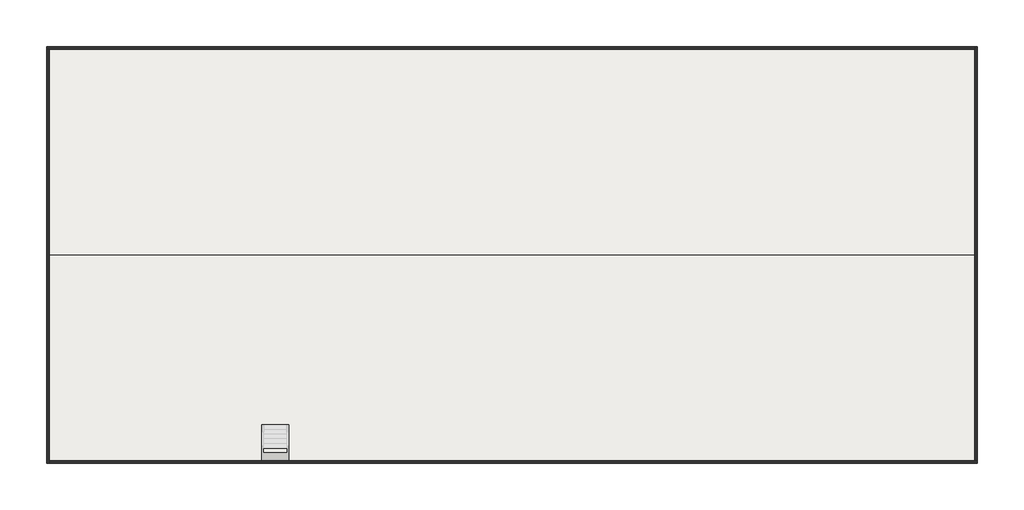
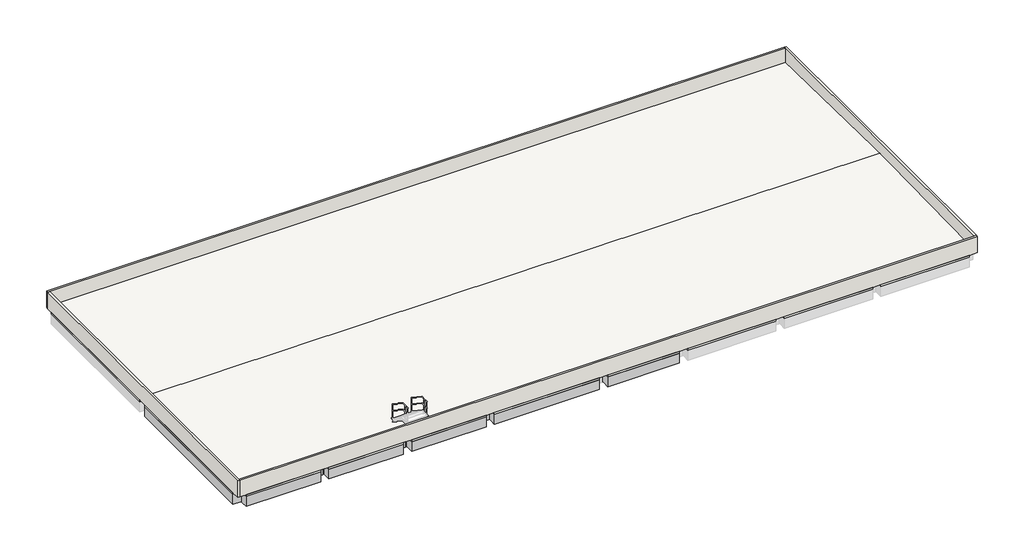
# One storey, part 1 of 3: 16 beams, 4 walls, 1 roof, 1 slab.
"""IFC4 building model written with IfcOpenShell, lengths in millimetres."""

import ifcopenshell
import ifcopenshell.guid

model = None  # the IFC model being written
_history = None  # IfcOwnerHistory: only IFC2X3 demands one
_inside = {}  # id of a spatial element -> (the spatial element, [elements in it])
_under = {}  # id of a project, library or spatial element -> (it, [spatial elements below it])
_declared = {}  # id of a project -> (the project, [libraries it declares])
_typed = {}  # id of a type object -> (the type object, [elements of that type])
_made_of = {}  # id of a material, layer set ... -> (it, [elements and type objects made of it])


def new_model(schema):
    """Start an empty IFC model of exactly this schema.

    Asked for "IFC4X3", IfcOpenShell would pick the latest addendum, in which some entities
    have other attributes; the version numbers below select the first issue.
    IFC2X3 requires an IfcOwnerHistory on every rooted entity: one is made here for all.
    """
    global model, _history
    if schema == "IFC4X3":
        model = ifcopenshell.file(schema_version=(4, 3, 0, 0))
    else:
        model = ifcopenshell.file(schema=schema)
    _inside.clear()
    _under.clear()
    _declared.clear()
    _typed.clear()
    _made_of.clear()
    _history = None
    if model.schema == "IFC2X3":
        org = make("IfcOrganization", Name="unknown")
        user = make(
            "IfcPersonAndOrganization",
            ThePerson=make("IfcPerson", FamilyName="unknown"),
            TheOrganization=org,
        )
        app = make(
            "IfcApplication",
            ApplicationDeveloper=org,
            Version="unknown",
            ApplicationFullName="unknown",
            ApplicationIdentifier="unknown",
        )
        _history = make(
            "IfcOwnerHistory",
            OwningUser=user,
            OwningApplication=app,
            ChangeAction="ADDED",
            CreationDate=0,
        )
    return model


def make(cls, **values):
    """One entity of the class cls with the attributes given. An attribute that is None is left unset."""
    return model.create_entity(
        cls, **{name: value for name, value in values.items() if value is not None}
    )


def rooted(cls, **values):
    """An entity with a GlobalId (a new one), such as an element, a storey or a relation."""
    return make(cls, GlobalId=ifcopenshell.guid.new(), OwnerHistory=_history, **values)


def si_unit(unit_type, name, prefix=None):
    """IfcSIUnit, for example si_unit("LENGTHUNIT", "METRE", prefix="MILLI")."""
    return make("IfcSIUnit", UnitType=unit_type, Prefix=prefix, Name=name)


def assignment(units):
    """IfcUnitAssignment: the units of a project."""
    return None if units is None else make("IfcUnitAssignment", Units=units)


def point(xyz):
    """IfcCartesianPoint."""
    return None if xyz is None else make("IfcCartesianPoint", Coordinates=xyz)


def direction(xyz):
    """IfcDirection."""
    return None if xyz is None else make("IfcDirection", DirectionRatios=xyz)


def frame(location, z_axis=None, x_axis=None):
    """IfcAxis2Placement3D, a coordinate frame: its origin and axes. An axis left out is left unset."""
    return make(
        "IfcAxis2Placement3D",
        Location=point(location),
        Axis=direction(z_axis),
        RefDirection=direction(x_axis),
    )


def origin():
    """The frame at (0, 0, 0) with its axes left unset."""
    return frame((0.0, 0.0, 0.0))


def place(relative_to, where):
    """IfcLocalPlacement: puts the frame where relative to a parent placement (None: the world)."""
    return make(
        "IfcLocalPlacement", PlacementRelTo=relative_to, RelativePlacement=where
    )


def context(
    kind, dimensions, precision=None, world=None, true_north=None, identifier=None
):
    """IfcGeometricRepresentationContext, for example the 3D "Model" context."""
    return make(
        "IfcGeometricRepresentationContext",
        ContextIdentifier=identifier,
        ContextType=kind,
        CoordinateSpaceDimension=dimensions,
        Precision=precision,
        WorldCoordinateSystem=world,
        TrueNorth=true_north,
    )


def project(units=None, contexts=None):
    """IfcProject with its units and contexts."""
    return rooted(
        "IfcProject",
        Name="project",
        RepresentationContexts=contexts,
        UnitsInContext=assignment(units),
    )


def spatial(cls, under=None, at=None, **own):
    """A site, building, storey or space (cls), placed at a placement, below another one or the project."""
    s = rooted(cls, ObjectPlacement=at, **own)
    if under is not None:
        _under.setdefault(under.id(), (under, []))[1].append(s)
    return s


def polyline(points):
    """IfcPolyline through the points."""
    return make("IfcPolyline", Points=[point(p) for p in points])


def outline(outer, holes=None, kind="AREA"):
    """IfcArbitraryClosedProfileDef: a profile drawn as a closed curve; with holes, ...WithVoids."""
    if holes is None:
        return make("IfcArbitraryClosedProfileDef", ProfileType=kind, OuterCurve=outer)
    return make(
        "IfcArbitraryProfileDefWithVoids",
        ProfileType=kind,
        OuterCurve=outer,
        InnerCurves=holes,
    )


def extrude(swept, where, along, depth):
    """IfcExtrudedAreaSolid: the profile swept, set in the frame where, extruded along a direction by depth."""
    return make(
        "IfcExtrudedAreaSolid",
        SweptArea=swept,
        Position=where,
        ExtrudedDirection=direction(along),
        Depth=depth,
    )


def faces_of(points, faces, orient=None, outer=None):
    """IfcFace entities. A face is a list of loops; a loop is a list of indices into points, from 0.

    orient and outer hold one flag for each loop. By default every Orientation is true, the
    first loop of a face is its IfcFaceOuterBound and the others are IfcFaceBound.
    """
    made = []
    for i, loops in enumerate(faces):
        bounds = []
        for j, loop in enumerate(loops):
            is_outer = j == 0 if outer is None else outer[i][j]
            bounds.append(
                make(
                    "IfcFaceOuterBound" if is_outer else "IfcFaceBound",
                    Bound=make("IfcPolyLoop", Polygon=[points[k] for k in loop]),
                    Orientation=True if orient is None else orient[i][j],
                )
            )
        made.append(make("IfcFace", Bounds=bounds))
    return made


def faceted_brep(points, faces, orient=None, outer=None, voids=None):
    """IfcFacetedBrep: a solid bounded by flat faces; with voids (closed shells), ...WithVoids."""
    shared = [point(p) for p in points]
    hull = make("IfcClosedShell", CfsFaces=faces_of(shared, faces, orient, outer))
    if voids is None:
        return make("IfcFacetedBrep", Outer=hull)
    return make(
        "IfcFacetedBrepWithVoids",
        Outer=hull,
        Voids=[
            make(cls, CfsFaces=faces_of(shared, fs, o, b)) for cls, fs, o, b in voids
        ],
    )


def shape(context_of_items, identifier, shape_type, items):
    """IfcShapeRepresentation: the items that make up one representation, for example the "Body"."""
    return make(
        "IfcShapeRepresentation",
        ContextOfItems=context_of_items,
        RepresentationIdentifier=identifier,
        RepresentationType=shape_type,
        Items=items,
    )


def made_of(thing, what):
    """Note that an element or type object is made of a material, layer set ...; save() writes the relation."""
    if what is not None:
        _made_of.setdefault(what.id(), (what, []))[1].append(thing)
    return thing


def element(
    cls,
    number,
    at=None,
    inside=None,
    cuts=None,
    type_object=None,
    material=None,
    context=None,
    identifier="Body",
    shape_type=None,
    held_by="IfcProductDefinitionShape",
    body=None,
    shapes=None,
    **own,
):
    """One element of the class cls, such as IfcWall. Its Tag is "e" and its number.

    at: its placement. inside: the storey or other place that contains it. cuts: it is an
    opening in that element (IfcRelVoidsElement). A single representation is given by context,
    identifier, shape_type and body (its items); several are given by shapes. held_by: the class
    of the entity that holds the representations. save() writes the other relations.
    """
    e = rooted(cls, Tag="e%d" % number, ObjectPlacement=at, **own)
    if body is not None:
        shapes = [shape(context, identifier, shape_type, body)]
    if shapes is not None:
        e.Representation = make(held_by, Representations=shapes)
    if inside is not None:
        _inside.setdefault(inside.id(), (inside, []))[1].append(e)
    if cuts is not None:
        rooted(
            "IfcRelVoidsElement", RelatingBuildingElement=cuts, RelatedOpeningElement=e
        )
    if type_object is not None:
        _typed.setdefault(type_object.id(), (type_object, []))[1].append(e)
    return made_of(e, material)


def aggregate(whole, parts):
    """IfcRelAggregates: a whole, such as a stair, and the parts it consists of."""
    return rooted("IfcRelAggregates", RelatingObject=whole, RelatedObjects=parts)


def save(model, path):
    """Write the relations noted so far, then the file.

    IfcRelAggregates (storeys below a building ...), IfcRelContainedInSpatialStructure (elements
    in a storey), IfcRelDefinesByType, IfcRelAssociatesMaterial and IfcRelDeclares: one each for
    every whole, place, type object, material and project.
    """
    for whole, parts in _under.values():
        aggregate(whole, parts)
    for where, things in _inside.values():
        rooted(
            "IfcRelContainedInSpatialStructure",
            RelatedElements=things,
            RelatingStructure=where,
        )
    for kind, things in _typed.values():
        rooted("IfcRelDefinesByType", RelatedObjects=things, RelatingType=kind)
    for what, things in _made_of.values():
        rooted("IfcRelAssociatesMaterial", RelatedObjects=things, RelatingMaterial=what)
    for by, libraries in _declared.values():
        rooted("IfcRelDeclares", RelatingContext=by, RelatedDefinitions=libraries)
    model.write(path)


model = new_model("IFC4")

# Units and contexts
model_context = context("Model", 3, world=origin())
ifc_project = project(units=[si_unit("LENGTHUNIT", "METRE", prefix="MILLI")], contexts=[model_context])

# Site, building, storey
site = spatial("IfcSite", under=ifc_project)
building = spatial("IfcBuilding", under=site)
storey = spatial("IfcBuildingStorey", under=building, Name="TOC", Elevation=7499.9618634)

# Beams
placement = place(None, origin())
element("IfcBeam", 1, ObjectType="RC Beam_Rectangular : H_SB_AR_S16_B600xH900_RG4", at=placement, inside=storey, context=model_context, shape_type="Brep", body=[
    faceted_brep([(300.0, 12499.5208589, 6599.9618634), (300.0, 12099.5208589, 6599.9618634), (300.0, 11899.5208589, 6599.9618634), (300.0, 11899.5208589, 7349.9618634), (300.0, 12499.5208589, 7349.9618634), (5700.0, 11899.5208589, 6599.9618634), (5700.0, 12099.5208589, 6599.9618634), (5700.0, 12499.5208589, 6599.9618634), (5700.0, 12499.5208589, 7349.9618634), (5700.0, 11899.5208589, 7349.9618634), (426.0, 11899.5208589, 7349.9618634), (2800.0, 11899.5208589, 7349.9618634), (3200.0, 11899.5208589, 7349.9618634), (3200.0, 12499.5208589, 7349.9618634), (2800.0, 12499.5208589, 7349.9618634), (426.0, 12499.5208589, 7349.9618634), (2800.0, 11899.5208589, 6599.9618634), (3200.0, 11899.5208589, 6599.9618634), (426.0, 12499.5208589, 6599.9618634), (2800.0, 12499.5208589, 6599.9618634), (3200.0, 12499.5208589, 6599.9618634)], [[[0, 1, 2, 3, 4]], [[5, 6, 7, 8, 9]], [[4, 3, 10, 11, 12, 9, 8, 13, 14, 15]], [[2, 16, 17, 5, 9, 12, 11, 10, 3]], [[2, 1, 0, 18, 19, 20, 7, 6, 5, 17, 16]], [[7, 20, 19, 18, 0, 4, 15, 14, 13, 8]]]),
])
element("IfcBeam", 2, ObjectType="RC Beam_Rectangular : H_SB_AR_S16_B600xH900_RG4", at=placement, inside=storey, context=model_context, shape_type="Brep", body=[
    faceted_brep([(6300.0, 12499.5208589, 6599.9618634), (6300.0, 12099.5208589, 6599.9618634), (6300.0, 11899.5208589, 6599.9618634), (6300.0, 11899.5208589, 7349.9618634), (6300.0, 12499.5208589, 7349.9618634), (11700.0, 11899.5208589, 6599.9618634), (11700.0, 12099.5208589, 6599.9618634), (11700.0, 12499.5208589, 6599.9618634), (11700.0, 12499.5208589, 7349.9618634), (11700.0, 11899.5208589, 7349.9618634), (8800.0, 11899.5208589, 7349.9618634), (9200.0, 11899.5208589, 7349.9618634), (9200.0, 12499.5208589, 7349.9618634), (8800.0, 12499.5208589, 7349.9618634), (8800.0, 11899.5208589, 6599.9618634), (9200.0, 11899.5208589, 6599.9618634), (8800.0, 12499.5208589, 6599.9618634), (9200.0, 12499.5208589, 6599.9618634)], [[[0, 1, 2, 3, 4]], [[5, 6, 7, 8, 9]], [[4, 3, 10, 11, 9, 8, 12, 13]], [[2, 14, 15, 5, 9, 11, 10, 3]], [[2, 1, 0, 16, 17, 7, 6, 5, 15, 14]], [[7, 17, 16, 0, 4, 13, 12, 8]]]),
])
element("IfcBeam", 3, ObjectType="RC Beam_Rectangular : H_SB_AR_S16_B600xH900_RG4", at=placement, inside=storey, context=model_context, shape_type="Brep", body=[
    faceted_brep([(12300.0, 12499.5208589, 6599.9618634), (12300.0, 12099.5208589, 6599.9618634), (12300.0, 11899.5208589, 6599.9618634), (12300.0, 11899.5208589, 7349.9618634), (12300.0, 12499.5208589, 7349.9618634), (17700.0, 11899.5208589, 6599.9618634), (17700.0, 12099.5208589, 6599.9618634), (17700.0, 12499.5208589, 6599.9618634), (17700.0, 12499.5208589, 7349.9618634), (17700.0, 11899.5208589, 7349.9618634), (14800.0, 11899.5208589, 7349.9618634), (15200.0, 11899.5208589, 7349.9618634), (15200.0, 12499.5208589, 7349.9618634), (14800.0, 12499.5208589, 7349.9618634), (14800.0, 11899.5208589, 6599.9618634), (15200.0, 11899.5208589, 6599.9618634), (14800.0, 12499.5208589, 6599.9618634), (15200.0, 12499.5208589, 6599.9618634)], [[[0, 1, 2, 3, 4]], [[5, 6, 7, 8, 9]], [[4, 3, 10, 11, 9, 8, 12, 13]], [[2, 14, 15, 5, 9, 11, 10, 3]], [[2, 1, 0, 16, 17, 7, 6, 5, 15, 14]], [[7, 17, 16, 0, 4, 13, 12, 8]]]),
])
element("IfcBeam", 4, ObjectType="RC Beam_Rectangular : H_SB_AR_S16_B600xH900_RG9", at=placement, inside=storey, context=model_context, shape_type="Brep", body=[
    faceted_brep([(300.0, 799.5208589, 6599.9618634), (300.0, 649.5208589, 6599.9618634), (300.0, 199.5208589, 6599.9618634), (300.0, 199.5208589, 7349.9618634), (300.0, 799.5208589, 7349.9618634), (5700.0, 199.5208589, 6599.9618634), (5700.0, 649.5208589, 6599.9618634), (5700.0, 799.5208589, 6599.9618634), (5700.0, 799.5208589, 7349.9618634), (5700.0, 199.5208589, 7349.9618634), (3200.0, 799.5208589, 7349.9618634), (2800.0, 799.5208589, 7349.9618634), (426.0, 799.5208589, 7349.9618634), (2800.0, 799.5208589, 6599.9618634), (3200.0, 799.5208589, 6599.9618634)], [[[0, 1, 2, 3, 4]], [[5, 6, 7, 8, 9]], [[4, 3, 9, 8, 10, 11, 12]], [[2, 5, 9, 3]], [[2, 1, 0, 13, 14, 7, 6, 5]], [[7, 14, 13, 0, 4, 12, 11, 10, 8]]]),
])
element("IfcBeam", 5, ObjectType="RC Beam_Rectangular : H_SB_AR_S16_B600xH900_RG9", at=placement, inside=storey, context=model_context, shape_type="Brep", body=[
    faceted_brep([(6300.0, 799.5208589, 6599.9618634), (6300.0, 649.5208589, 6599.9618634), (6300.0, 199.5208589, 6599.9618634), (6300.0, 199.5208589, 7349.9618634), (6300.0, 799.5208589, 7349.9618634), (11700.0, 199.5208589, 6599.9618634), (11700.0, 649.5208589, 6599.9618634), (11700.0, 799.5208589, 6599.9618634), (11700.0, 799.5208589, 7349.9618634), (11700.0, 199.5208589, 7349.9618634), (9200.0, 799.5208589, 7349.9618634), (8800.0, 799.5208589, 7349.9618634), (8800.0, 799.5208589, 6599.9618634), (9200.0, 799.5208589, 6599.9618634)], [[[0, 1, 2, 3, 4]], [[5, 6, 7, 8, 9]], [[4, 3, 9, 8, 10, 11]], [[2, 5, 9, 3]], [[2, 1, 0, 12, 13, 7, 6, 5]], [[7, 13, 12, 0, 4, 11, 10, 8]]]),
])
element("IfcBeam", 6, ObjectType="RC Beam_Rectangular : H_SB_AR_S16_B600xH900_RG9", at=placement, inside=storey, context=model_context, shape_type="Brep", body=[
    faceted_brep([(12300.0, 799.5208589, 6599.9618634), (12300.0, 649.5208589, 6599.9618634), (12300.0, 199.5208589, 6599.9618634), (12300.0, 199.5208589, 7349.9618634), (12300.0, 799.5208589, 7349.9618634), (17700.0, 199.5208589, 6599.9618634), (17700.0, 649.5208589, 6599.9618634), (17700.0, 799.5208589, 6599.9618634), (17700.0, 799.5208589, 7349.9618634), (17700.0, 199.5208589, 7349.9618634), (15200.0, 799.5208589, 7349.9618634), (14800.0, 799.5208589, 7349.9618634), (14800.0, 799.5208589, 6599.9618634), (15200.0, 799.5208589, 6599.9618634)], [[[0, 1, 2, 3, 4]], [[5, 6, 7, 8, 9]], [[4, 3, 9, 8, 10, 11]], [[2, 5, 9, 3]], [[2, 1, 0, 12, 13, 7, 6, 5]], [[7, 13, 12, 0, 4, 11, 10, 8]]]),
])
element("IfcBeam", 7, ObjectType="RC Beam_Rectangular : H_SB_AR_S16_B600xH900_RG9", at=placement, inside=storey, context=model_context, shape_type="Brep", body=[
    faceted_brep([(18300.0, 799.5208589, 6599.9618634), (18300.0, 649.5208589, 6599.9618634), (18300.0, 199.5208589, 6599.9618634), (18300.0, 199.5208589, 7349.9618634), (18300.0, 799.5208589, 7349.9618634), (25900.0, 199.5208589, 6599.9618634), (25900.0, 649.5208589, 6599.9618634), (25900.0, 799.5208589, 6599.9618634), (25900.0, 799.5208589, 7349.9618634), (25900.0, 199.5208589, 7349.9618634), (22400.0, 799.5208589, 7349.9618634), (21800.0, 799.5208589, 7349.9618634), (21800.0, 799.5208589, 6599.9618634), (22400.0, 799.5208589, 6599.9618634)], [[[0, 1, 2, 3, 4]], [[5, 6, 7, 8, 9]], [[4, 3, 9, 8, 10, 11]], [[2, 5, 9, 3]], [[2, 1, 0, 12, 13, 7, 6, 5]], [[7, 13, 12, 0, 4, 11, 10, 8]]]),
])
element("IfcBeam", 8, ObjectType="RC Beam_Rectangular : H_SB_AR_S16_B600xH900_RG9", at=placement, inside=storey, context=model_context, shape_type="Brep", body=[
    faceted_brep([(26500.0, 799.5208589, 6599.9618634), (26500.0, 649.5208589, 6599.9618634), (26500.0, 199.5208589, 6599.9618634), (26500.0, 199.5208589, 7349.9618634), (26500.0, 799.5208589, 7349.9618634), (31700.0, 199.5208589, 6599.9618634), (31700.0, 649.5208589, 6599.9618634), (31700.0, 799.5208589, 6599.9618634), (31700.0, 799.5208589, 7349.9618634), (31700.0, 199.5208589, 7349.9618634), (29400.0, 799.5208589, 7349.9618634), (28800.0, 799.5208589, 7349.9618634), (28700.0, 799.5208589, 7349.9618634), (28500.0, 799.5208589, 7349.9618634), (27855.0, 799.5208589, 7349.9618634), (26724.0, 799.5208589, 7349.9618634), (28800.0, 799.5208589, 6599.9618634), (29400.0, 799.5208589, 6599.9618634)], [[[0, 1, 2, 3, 4]], [[5, 6, 7, 8, 9]], [[4, 3, 9, 8, 10, 11, 12, 13, 14, 15]], [[2, 5, 9, 3]], [[2, 1, 0, 16, 17, 7, 6, 5]], [[7, 17, 16, 0, 4, 15, 14, 13, 12, 11, 10, 8]]]),
])
element("IfcBeam", 9, ObjectType="RC Beam_Rectangular : H_SB_AR_S16_B600xH900_RG6", at=placement, inside=storey, context=model_context, shape_type="Brep", body=[
    faceted_brep([(300.0, 11899.5208589, 6599.9618634), (150.0, 11899.5208589, 6599.9618634), (-300.0, 11899.5208589, 6599.9618634), (-300.0, 11899.5208589, 7349.9618634), (300.0, 11899.5208589, 7349.9618634), (-300.0, 799.5208589, 6599.9618634), (150.0, 799.5208589, 6599.9618634), (300.0, 799.5208589, 6599.9618634), (300.0, 799.5208589, 7349.9618634), (-300.0, 799.5208589, 7349.9618634)], [[[0, 1, 2, 3, 4]], [[5, 6, 7, 8, 9]], [[4, 3, 9, 8]], [[7, 0, 4, 8]], [[2, 1, 0, 7, 6, 5]], [[2, 5, 9, 3]]]),
])
element("IfcBeam", 10, ObjectType="RC Beam_Rectangular : H_SB_AR_S16_B400xH900_RG1", at=placement, inside=storey, context=model_context, shape_type="Brep", body=[
    faceted_brep([(5800.0, 799.5208589, 7349.9618634), (6200.0, 799.5208589, 7349.9618634), (6200.0, 925.5208589, 7349.9618634), (6200.0, 11899.5208589, 7349.9618634), (5800.0, 11899.5208589, 7349.9618634), (5800.0, 925.5208589, 7349.9618634), (5800.0, 799.5208589, 6599.9618634), (6200.0, 799.5208589, 6599.9618634), (6200.0, 11899.5208589, 6599.9618634), (5800.0, 11899.5208589, 6599.9618634), (6200.0, 925.5208589, 6599.9618634), (5800.0, 925.5208589, 6599.9618634)], [[[0, 1, 2, 3, 4, 5]], [[6, 7, 1, 0]], [[8, 9, 4, 3]], [[7, 10, 8, 3, 2, 1]], [[6, 11, 9, 8, 10, 7]], [[9, 11, 6, 0, 5, 4]]]),
])
element("IfcBeam", 11, ObjectType="RC Beam_Rectangular : H_SB_AR_S16_B400xH900_RG1", at=placement, inside=storey, context=model_context, shape_type="Brep", body=[
    faceted_brep([(11800.0, 799.5208589, 7349.9618634), (12200.0, 799.5208589, 7349.9618634), (12200.0, 925.5208589, 7349.9618634), (12200.0, 11899.5208589, 7349.9618634), (11800.0, 11899.5208589, 7349.9618634), (11800.0, 925.5208589, 7349.9618634), (11800.0, 799.5208589, 6599.9618634), (12200.0, 799.5208589, 6599.9618634), (12200.0, 11899.5208589, 6599.9618634), (11800.0, 11899.5208589, 6599.9618634), (12200.0, 925.5208589, 6599.9618634), (11800.0, 925.5208589, 6599.9618634)], [[[0, 1, 2, 3, 4, 5]], [[6, 7, 1, 0]], [[8, 9, 4, 3]], [[7, 10, 8, 3, 2, 1]], [[6, 11, 9, 8, 10, 7]], [[9, 11, 6, 0, 5, 4]]]),
])
element("IfcBeam", 12, ObjectType="RC Beam_Rectangular : H_SB_AR_S16_B600xH900_RG1A", at=placement, inside=storey, context=model_context, shape_type="Brep", body=[
    faceted_brep([(17700.0, 799.5208589, 7349.9618634), (18300.0, 799.5208589, 7349.9618634), (18300.0, 925.5208589, 7349.9618634), (18300.0, 7999.5208589, 7349.9618634), (18300.0, 8599.5208589, 7349.9618634), (18300.0, 11899.5208589, 7349.9618634), (17700.0, 11899.5208589, 7349.9618634), (17700.0, 925.5208589, 7349.9618634), (17700.0, 799.5208589, 6599.9618634), (18100.0, 799.5208589, 6599.9618634), (18300.0, 799.5208589, 6599.9618634), (18300.0, 11899.5208589, 6599.9618634), (18100.0, 11899.5208589, 6599.9618634), (17700.0, 11899.5208589, 6599.9618634), (18300.0, 7999.5208589, 6599.9618634), (18300.0, 8599.5208589, 6599.9618634), (17700.0, 925.5208589, 6599.9618634)], [[[0, 1, 2, 3, 4, 5, 6, 7]], [[8, 9, 10, 1, 0]], [[11, 12, 13, 6, 5]], [[10, 14, 15, 11, 5, 4, 3, 2, 1]], [[8, 16, 13, 12, 11, 15, 14, 10, 9]], [[13, 16, 8, 0, 7, 6]]]),
])
element("IfcBeam", 13, ObjectType="RC Beam_Rectangular : H_SB_AR_S16_B400xH900_RB1", at=placement, inside=storey, context=model_context, shape_type="Brep", body=[
    faceted_brep([(2800.0, 11899.5208589, 6599.9618634), (2800.0, 925.5208589, 6599.9618634), (2800.0, 799.5208589, 6599.9618634), (2800.0, 799.5208589, 7349.9618634), (2800.0, 925.5208589, 7349.9618634), (2800.0, 11899.5208589, 7349.9618634), (3200.0, 11899.5208589, 6599.9618634), (3200.0, 925.5208589, 6599.9618634), (3200.0, 799.5208589, 6599.9618634), (3200.0, 11899.5208589, 7349.9618634), (3200.0, 925.5208589, 7349.9618634), (3200.0, 799.5208589, 7349.9618634)], [[[0, 1, 2, 3, 4, 5]], [[0, 6, 7, 8, 2, 1]], [[8, 7, 6, 9, 10, 11]], [[6, 0, 5, 9]], [[2, 8, 11, 3]], [[5, 4, 3, 11, 10, 9]]]),
])
element("IfcBeam", 14, ObjectType="RC Beam_Rectangular : H_SB_AR_S16_B400xH900_RB1", at=placement, inside=storey, context=model_context, shape_type="Brep", body=[
    faceted_brep([(8800.0, 11899.5208589, 6599.9618634), (8800.0, 925.5208589, 6599.9618634), (8800.0, 799.5208589, 6599.9618634), (8800.0, 799.5208589, 7349.9618634), (8800.0, 925.5208589, 7349.9618634), (8800.0, 11899.5208589, 7349.9618634), (9200.0, 11899.5208589, 6599.9618634), (9200.0, 925.5208589, 6599.9618634), (9200.0, 799.5208589, 6599.9618634), (9200.0, 11899.5208589, 7349.9618634), (9200.0, 925.5208589, 7349.9618634), (9200.0, 799.5208589, 7349.9618634)], [[[0, 1, 2, 3, 4, 5]], [[0, 6, 7, 8, 2, 1]], [[8, 7, 6, 9, 10, 11]], [[6, 0, 5, 9]], [[2, 8, 11, 3]], [[5, 4, 3, 11, 10, 9]]]),
])
element("IfcBeam", 15, ObjectType="RC Beam_Rectangular : H_SB_AR_S16_B400xH900_RB1", at=placement, inside=storey, context=model_context, shape_type="Brep", body=[
    faceted_brep([(14800.0, 11899.5208589, 6599.9618634), (14800.0, 925.5208589, 6599.9618634), (14800.0, 799.5208589, 6599.9618634), (14800.0, 799.5208589, 7349.9618634), (14800.0, 925.5208589, 7349.9618634), (14800.0, 11899.5208589, 7349.9618634), (15200.0, 11899.5208589, 6599.9618634), (15200.0, 925.5208589, 6599.9618634), (15200.0, 799.5208589, 6599.9618634), (15200.0, 11899.5208589, 7349.9618634), (15200.0, 925.5208589, 7349.9618634), (15200.0, 799.5208589, 7349.9618634)], [[[0, 1, 2, 3, 4, 5]], [[0, 6, 7, 8, 2, 1]], [[8, 7, 6, 9, 10, 11]], [[6, 0, 5, 9]], [[2, 8, 11, 3]], [[5, 4, 3, 11, 10, 9]]]),
])
element("IfcBeam", 16, ObjectType="RC Beam_Rectangular : H_SB_AR_S16_B600xH900_RB3", at=placement, inside=storey, context=model_context, shape_type="Brep", body=[
    faceted_brep([(21800.0, 7999.5208589, 6599.9618634), (21800.0, 925.5208589, 6599.9618634), (21800.0, 799.5208589, 6599.9618634), (21800.0, 799.5208589, 7349.9618634), (21800.0, 925.5208589, 7349.9618634), (21800.0, 7999.5208589, 7349.9618634), (22400.0, 7999.5208589, 6599.9618634), (22400.0, 925.5208589, 6599.9618634), (22400.0, 799.5208589, 6599.9618634), (22400.0, 7999.5208589, 7349.9618634), (22400.0, 925.5208589, 7349.9618634), (22400.0, 799.5208589, 7349.9618634)], [[[0, 1, 2, 3, 4, 5]], [[0, 6, 7, 8, 2, 1]], [[8, 7, 6, 9, 10, 11]], [[6, 0, 5, 9]], [[2, 8, 11, 3]], [[5, 4, 3, 11, 10, 9]]]),
])

# Roof
element("IfcRoof", 17, ObjectType="H_RF_AR_B06_Mortar(Slope)_XPS_Memb_T50+120", at=placement, inside=storey, context=model_context, shape_type="SweptSolid", body=[
    extrude(outline(polyline([(24049.5208589, 7671.4618634), (24049.5208589, 7499.9618634), (349.5208589, 7499.9618634), (349.5208589, 7671.4618634), (12199.5208589, 7904.4618634), (24049.5208589, 7671.4618634)])), frame((-150.0, 0.0, 0.0), z_axis=(1.0, 0.0, 0.0), x_axis=(0.0, 1.0, 0.0)), (0.0, 0.0, 1.0), 53300.0),
])

# Slab
element("IfcSlab", 18, ObjectType="H_FL_AR_S17_Roof RC Slab_T150", at=placement, inside=storey, context=model_context, shape_type="Brep", body=[
    faceted_brep([(300.0, 11899.5208589, 7349.9618634), (300.0, 12499.5208589, 7349.9618634), (-300.0, 12499.5208589, 7349.9618634), (-300.0, 23599.5208589, 7349.9618634), (300.0, 23599.5208589, 7349.9618634), (300.0, 24199.5208589, 7349.9618634), (5700.0, 24199.5208589, 7349.9618634), (5700.0, 23599.5208589, 7349.9618634), (5800.0, 23599.5208589, 7349.9618634), (6200.0, 23599.5208589, 7349.9618634), (6300.0, 23599.5208589, 7349.9618634), (6300.0, 24199.5208589, 7349.9618634), (11700.0, 24199.5208589, 7349.9618634), (11700.0, 23599.5208589, 7349.9618634), (11800.0, 23599.5208589, 7349.9618634), (12200.0, 23599.5208589, 7349.9618634), (12300.0, 23599.5208589, 7349.9618634), (12300.0, 24199.5208589, 7349.9618634), (17700.0, 24199.5208589, 7349.9618634), (17700.0, 23599.5208589, 7349.9618634), (18300.0, 23599.5208589, 7349.9618634), (18300.0, 24199.5208589, 7349.9618634), (25900.0, 24199.5208589, 7349.9618634), (25900.0, 23599.5208589, 7349.9618634), (25950.0, 23599.5208589, 7349.9618634), (26450.0, 23599.5208589, 7349.9618634), (26500.0, 23599.5208589, 7349.9618634), (26500.0, 24199.5208589, 7349.9618634), (31700.0, 24199.5208589, 7349.9618634), (31700.0, 23599.5208589, 7349.9618634), (31750.0, 23599.5208589, 7349.9618634), (32250.0, 23599.5208589, 7349.9618634), (32300.0, 23599.5208589, 7349.9618634), (32300.0, 24199.5208589, 7349.9618634), (38700.0, 24199.5208589, 7349.9618634), (38700.0, 23599.5208589, 7349.9618634), (38750.0, 23599.5208589, 7349.9618634), (39250.0, 23599.5208589, 7349.9618634), (39300.0, 23599.5208589, 7349.9618634), (39300.0, 24199.5208589, 7349.9618634), (45700.0, 24199.5208589, 7349.9618634), (45700.0, 23599.5208589, 7349.9618634), (45750.0, 23599.5208589, 7349.9618634), (46250.0, 23599.5208589, 7349.9618634), (46300.0, 23599.5208589, 7349.9618634), (46300.0, 24199.5208589, 7349.9618634), (52700.0, 24199.5208589, 7349.9618634), (52700.0, 23599.5208589, 7349.9618634), (53300.0, 23599.5208589, 7349.9618634), (53300.0, 8599.5208589, 7349.9618634), (52700.0, 8599.5208589, 7349.9618634), (52700.0, 7999.5208589, 7349.9618634), (53300.0, 7999.5208589, 7349.9618634), (53300.0, 799.5208589, 7349.9618634), (52700.0, 799.5208589, 7349.9618634), (52700.0, 199.5208589, 7349.9618634), (46300.0, 199.5208589, 7349.9618634), (46300.0, 799.5208589, 7349.9618634), (46250.0, 799.5208589, 7349.9618634), (45750.0, 799.5208589, 7349.9618634), (45700.0, 799.5208589, 7349.9618634), (45700.0, 199.5208589, 7349.9618634), (39300.0, 199.5208589, 7349.9618634), (39300.0, 799.5208589, 7349.9618634), (39250.0, 799.5208589, 7349.9618634), (38750.0, 799.5208589, 7349.9618634), (38700.0, 799.5208589, 7349.9618634), (38700.0, 199.5208589, 7349.9618634), (32300.0, 199.5208589, 7349.9618634), (32300.0, 799.5208589, 7349.9618634), (32250.0, 799.5208589, 7349.9618634), (31750.0, 799.5208589, 7349.9618634), (31700.0, 799.5208589, 7349.9618634), (31700.0, 199.5208589, 7349.9618634), (26500.0, 199.5208589, 7349.9618634), (26500.0, 799.5208589, 7349.9618634), (26450.0, 799.5208589, 7349.9618634), (25950.0, 799.5208589, 7349.9618634), (25900.0, 799.5208589, 7349.9618634), (25900.0, 199.5208589, 7349.9618634), (18300.0, 199.5208589, 7349.9618634), (18300.0, 799.5208589, 7349.9618634), (17700.0, 799.5208589, 7349.9618634), (17700.0, 199.5208589, 7349.9618634), (12300.0, 199.5208589, 7349.9618634), (12300.0, 799.5208589, 7349.9618634), (12200.0, 799.5208589, 7349.9618634), (11800.0, 799.5208589, 7349.9618634), (11700.0, 799.5208589, 7349.9618634), (11700.0, 199.5208589, 7349.9618634), (6300.0, 199.5208589, 7349.9618634), (6300.0, 799.5208589, 7349.9618634), (6200.0, 799.5208589, 7349.9618634), (5800.0, 799.5208589, 7349.9618634), (5700.0, 799.5208589, 7349.9618634), (5700.0, 199.5208589, 7349.9618634), (300.0, 199.5208589, 7349.9618634), (300.0, 799.5208589, 7349.9618634), (-300.0, 799.5208589, 7349.9618634), (-300.0, 11899.5208589, 7349.9618634), (18300.0, 11899.5208589, 7349.9618634), (18300.0, 12499.5208589, 7349.9618634), (17700.0, 12499.5208589, 7349.9618634), (17700.0, 11899.5208589, 7349.9618634), (6300.0, 11899.5208589, 7349.9618634), (6300.0, 12499.5208589, 7349.9618634), (6200.0, 12499.5208589, 7349.9618634), (5800.0, 12499.5208589, 7349.9618634), (5700.0, 12499.5208589, 7349.9618634), (5700.0, 11899.5208589, 7349.9618634), (5800.0, 11899.5208589, 7349.9618634), (6200.0, 11899.5208589, 7349.9618634), (12300.0, 11899.5208589, 7349.9618634), (12300.0, 12499.5208589, 7349.9618634), (12200.0, 12499.5208589, 7349.9618634), (11800.0, 12499.5208589, 7349.9618634), (11700.0, 12499.5208589, 7349.9618634), (11700.0, 11899.5208589, 7349.9618634), (11800.0, 11899.5208589, 7349.9618634), (12200.0, 11899.5208589, 7349.9618634), (26500.0, 7999.5208589, 7349.9618634), (26500.0, 8599.5208589, 7349.9618634), (26450.0, 8599.5208589, 7349.9618634), (25950.0, 8599.5208589, 7349.9618634), (25900.0, 8599.5208589, 7349.9618634), (25900.0, 7999.5208589, 7349.9618634), (25950.0, 7999.5208589, 7349.9618634), (26450.0, 7999.5208589, 7349.9618634), (32300.0, 7999.5208589, 7349.9618634), (32300.0, 8599.5208589, 7349.9618634), (32250.0, 8599.5208589, 7349.9618634), (31750.0, 8599.5208589, 7349.9618634), (31700.0, 8599.5208589, 7349.9618634), (31700.0, 7999.5208589, 7349.9618634), (31750.0, 7999.5208589, 7349.9618634), (32250.0, 7999.5208589, 7349.9618634), (39300.0, 7999.5208589, 7349.9618634), (39300.0, 8599.5208589, 7349.9618634), (39250.0, 8599.5208589, 7349.9618634), (38750.0, 8599.5208589, 7349.9618634), (38700.0, 8599.5208589, 7349.9618634), (38700.0, 7999.5208589, 7349.9618634), (38750.0, 7999.5208589, 7349.9618634), (39250.0, 7999.5208589, 7349.9618634), (46300.0, 7999.5208589, 7349.9618634), (46300.0, 8599.5208589, 7349.9618634), (46250.0, 8599.5208589, 7349.9618634), (45750.0, 8599.5208589, 7349.9618634), (45700.0, 8599.5208589, 7349.9618634), (45700.0, 7999.5208589, 7349.9618634), (45750.0, 7999.5208589, 7349.9618634), (46250.0, 7999.5208589, 7349.9618634), (300.0, 12499.5208589, 7499.9618634), (300.0, 11899.5208589, 7499.9618634), (-300.0, 11899.5208589, 7499.9618634), (-300.0, 799.5208589, 7499.9618634), (300.0, 799.5208589, 7499.9618634), (300.0, 199.5208589, 7499.9618634), (5700.0, 199.5208589, 7499.9618634), (5700.0, 799.5208589, 7499.9618634), (6300.0, 799.5208589, 7499.9618634), (6300.0, 199.5208589, 7499.9618634), (11700.0, 199.5208589, 7499.9618634), (11700.0, 799.5208589, 7499.9618634), (12300.0, 799.5208589, 7499.9618634), (12300.0, 199.5208589, 7499.9618634), (17700.0, 199.5208589, 7499.9618634), (17700.0, 799.5208589, 7499.9618634), (18300.0, 799.5208589, 7499.9618634), (18300.0, 199.5208589, 7499.9618634), (25900.0, 199.5208589, 7499.9618634), (25900.0, 799.5208589, 7499.9618634), (26500.0, 799.5208589, 7499.9618634), (26500.0, 199.5208589, 7499.9618634), (31700.0, 199.5208589, 7499.9618634), (31700.0, 799.5208589, 7499.9618634), (32300.0, 799.5208589, 7499.9618634), (32300.0, 199.5208589, 7499.9618634), (38700.0, 199.5208589, 7499.9618634), (38700.0, 799.5208589, 7499.9618634), (39300.0, 799.5208589, 7499.9618634), (39300.0, 199.5208589, 7499.9618634), (45700.0, 199.5208589, 7499.9618634), (45700.0, 799.5208589, 7499.9618634), (46300.0, 799.5208589, 7499.9618634), (46300.0, 199.5208589, 7499.9618634), (52700.0, 199.5208589, 7499.9618634), (52700.0, 799.5208589, 7499.9618634), (53300.0, 799.5208589, 7499.9618634), (53300.0, 7999.5208589, 7499.9618634), (52700.0, 7999.5208589, 7499.9618634), (52700.0, 8599.5208589, 7499.9618634), (53300.0, 8599.5208589, 7499.9618634), (53300.0, 23599.5208589, 7499.9618634), (52700.0, 23599.5208589, 7499.9618634), (52700.0, 24199.5208589, 7499.9618634), (46300.0, 24199.5208589, 7499.9618634), (46300.0, 23599.5208589, 7499.9618634), (45700.0, 23599.5208589, 7499.9618634), (45700.0, 24199.5208589, 7499.9618634), (39300.0, 24199.5208589, 7499.9618634), (39300.0, 23599.5208589, 7499.9618634), (38700.0, 23599.5208589, 7499.9618634), (38700.0, 24199.5208589, 7499.9618634), (32300.0, 24199.5208589, 7499.9618634), (32300.0, 23599.5208589, 7499.9618634), (31700.0, 23599.5208589, 7499.9618634), (31700.0, 24199.5208589, 7499.9618634), (26500.0, 24199.5208589, 7499.9618634), (26500.0, 23599.5208589, 7499.9618634), (25900.0, 23599.5208589, 7499.9618634), (25900.0, 24199.5208589, 7499.9618634), (18300.0, 24199.5208589, 7499.9618634), (18300.0, 23599.5208589, 7499.9618634), (17700.0, 23599.5208589, 7499.9618634), (17700.0, 24199.5208589, 7499.9618634), (12300.0, 24199.5208589, 7499.9618634), (12300.0, 23599.5208589, 7499.9618634), (11700.0, 23599.5208589, 7499.9618634), (11700.0, 24199.5208589, 7499.9618634), (6300.0, 24199.5208589, 7499.9618634), (6300.0, 23599.5208589, 7499.9618634), (5700.0, 23599.5208589, 7499.9618634), (5700.0, 24199.5208589, 7499.9618634), (300.0, 24199.5208589, 7499.9618634), (300.0, 23599.5208589, 7499.9618634), (-300.0, 23599.5208589, 7499.9618634), (-300.0, 12499.5208589, 7499.9618634), (6300.0, 12499.5208589, 7499.9618634), (6300.0, 11899.5208589, 7499.9618634), (5700.0, 11899.5208589, 7499.9618634), (5700.0, 12499.5208589, 7499.9618634), (12300.0, 12499.5208589, 7499.9618634), (12300.0, 11899.5208589, 7499.9618634), (11700.0, 11899.5208589, 7499.9618634), (11700.0, 12499.5208589, 7499.9618634), (18300.0, 12499.5208589, 7499.9618634), (18300.0, 11899.5208589, 7499.9618634), (17700.0, 11899.5208589, 7499.9618634), (17700.0, 12499.5208589, 7499.9618634), (26500.0, 8599.5208589, 7499.9618634), (26500.0, 7999.5208589, 7499.9618634), (25900.0, 7999.5208589, 7499.9618634), (25900.0, 8599.5208589, 7499.9618634), (32300.0, 8599.5208589, 7499.9618634), (32300.0, 7999.5208589, 7499.9618634), (31700.0, 7999.5208589, 7499.9618634), (31700.0, 8599.5208589, 7499.9618634), (39300.0, 8599.5208589, 7499.9618634), (39300.0, 7999.5208589, 7499.9618634), (38700.0, 7999.5208589, 7499.9618634), (38700.0, 8599.5208589, 7499.9618634), (46300.0, 8599.5208589, 7499.9618634), (46300.0, 7999.5208589, 7499.9618634), (45700.0, 7999.5208589, 7499.9618634), (45700.0, 8599.5208589, 7499.9618634)], [[[0, 1, 2, 3, 4, 5, 6, 7, 8, 9, 10, 11, 12, 13, 14, 15, 16, 17, 18, 19, 20, 21, 22, 23, 24, 25, 26, 27, 28, 29, 30, 31, 32, 33, 34, 35, 36, 37, 38, 39, 40, 41, 42, 43, 44, 45, 46, 47, 48, 49, 50, 51, 52, 53, 54, 55, 56, 57, 58, 59, 60, 61, 62, 63, 64, 65, 66, 67, 68, 69, 70, 71, 72, 73, 74, 75, 76, 77, 78, 79, 80, 81, 82, 83, 84, 85, 86, 87, 88, 89, 90, 91, 92, 93, 94, 95, 96, 97, 98, 99], [100, 101, 102, 103], [104, 105, 106, 107, 108, 109, 110, 111], [112, 113, 114, 115, 116, 117, 118, 119], [120, 121, 122, 123, 124, 125, 126, 127], [128, 129, 130, 131, 132, 133, 134, 135], [136, 137, 138, 139, 140, 141, 142, 143], [144, 145, 146, 147, 148, 149, 150, 151]], [[152, 153, 154, 155, 156, 157, 158, 159, 160, 161, 162, 163, 164, 165, 166, 167, 168, 169, 170, 171, 172, 173, 174, 175, 176, 177, 178, 179, 180, 181, 182, 183, 184, 185, 186, 187, 188, 189, 190, 191, 192, 193, 194, 195, 196, 197, 198, 199, 200, 201, 202, 203, 204, 205, 206, 207, 208, 209, 210, 211, 212, 213, 214, 215, 216, 217, 218, 219, 220, 221, 222, 223, 224, 225, 226, 227], [228, 229, 230, 231], [232, 233, 234, 235], [236, 237, 238, 239], [240, 241, 242, 243], [244, 245, 246, 247], [248, 249, 250, 251], [252, 253, 254, 255]], [[48, 193, 192, 49]], [[52, 189, 188, 53]], [[157, 96, 95, 158]], [[161, 90, 89, 162]], [[165, 84, 83, 166]], [[169, 80, 79, 170]], [[173, 74, 73, 174]], [[177, 68, 67, 178]], [[181, 62, 61, 182]], [[185, 56, 55, 186]], [[154, 99, 98, 155]], [[2, 227, 226, 3]], [[5, 224, 223, 6]], [[11, 220, 219, 12]], [[17, 216, 215, 18]], [[21, 212, 211, 22]], [[27, 208, 207, 28]], [[33, 204, 203, 34]], [[39, 200, 199, 40]], [[45, 196, 195, 46]], [[0, 153, 152, 1]], [[153, 0, 99, 154]], [[1, 152, 227, 2]], [[104, 229, 228, 105]], [[229, 104, 111, 110, 109, 230]], [[230, 109, 108, 231]], [[231, 108, 107, 106, 105, 228]], [[112, 233, 232, 113]], [[233, 112, 119, 118, 117, 234]], [[234, 117, 116, 235]], [[235, 116, 115, 114, 113, 232]], [[100, 237, 236, 101]], [[237, 100, 103, 238]], [[238, 103, 102, 239]], [[239, 102, 101, 236]], [[4, 225, 224, 5]], [[225, 4, 3, 226]], [[10, 221, 220, 11]], [[221, 10, 9, 8, 7, 222]], [[222, 7, 6, 223]], [[16, 217, 216, 17]], [[217, 16, 15, 14, 13, 218]], [[218, 13, 12, 219]], [[20, 213, 212, 21]], [[213, 20, 19, 214]], [[214, 19, 18, 215]], [[26, 209, 208, 27]], [[209, 26, 25, 24, 23, 210]], [[210, 23, 22, 211]], [[32, 205, 204, 33]], [[205, 32, 31, 30, 29, 206]], [[206, 29, 28, 207]], [[38, 201, 200, 39]], [[201, 38, 37, 36, 35, 202]], [[202, 35, 34, 203]], [[44, 197, 196, 45]], [[197, 44, 43, 42, 41, 198]], [[198, 41, 40, 199]], [[47, 194, 193, 48]], [[194, 47, 46, 195]], [[120, 241, 240, 121]], [[241, 120, 127, 126, 125, 242]], [[242, 125, 124, 243]], [[243, 124, 123, 122, 121, 240]], [[128, 245, 244, 129]], [[245, 128, 135, 134, 133, 246]], [[246, 133, 132, 247]], [[247, 132, 131, 130, 129, 244]], [[136, 249, 248, 137]], [[249, 136, 143, 142, 141, 250]], [[250, 141, 140, 251]], [[251, 140, 139, 138, 137, 248]], [[144, 253, 252, 145]], [[253, 144, 151, 150, 149, 254]], [[254, 149, 148, 255]], [[255, 148, 147, 146, 145, 252]], [[51, 190, 189, 52]], [[190, 51, 50, 191]], [[191, 50, 49, 192]], [[156, 97, 96, 157]], [[97, 156, 155, 98]], [[160, 91, 90, 161]], [[94, 159, 158, 95]], [[159, 94, 93, 92, 91, 160]], [[164, 85, 84, 165]], [[88, 163, 162, 89]], [[163, 88, 87, 86, 85, 164]], [[168, 81, 80, 169]], [[82, 167, 166, 83]], [[167, 82, 81, 168]], [[172, 75, 74, 173]], [[78, 171, 170, 79]], [[171, 78, 77, 76, 75, 172]], [[176, 69, 68, 177]], [[72, 175, 174, 73]], [[175, 72, 71, 70, 69, 176]], [[180, 63, 62, 181]], [[66, 179, 178, 67]], [[179, 66, 65, 64, 63, 180]], [[184, 57, 56, 185]], [[60, 183, 182, 61]], [[183, 60, 59, 58, 57, 184]], [[54, 187, 186, 55]], [[187, 54, 53, 188]]]),
])

# Walls
element("IfcWall", 19, ObjectType="H_WA_AR_B02_Ext Wall_RC T150", at=placement, inside=storey, context=model_context, shape_type="Brep", body=[
    faceted_brep([(-300.0, 24049.5208589, 7499.9618634), (-150.0, 24049.5208589, 7499.9618634), (53150.0, 24049.5208589, 7499.9618634), (53150.0, 24049.5208589, 7671.4618634), (53150.0, 24049.5208589, 8749.9618634), (-150.0, 24049.5208589, 8749.9618634), (-300.0, 24049.5208589, 8749.9618634), (-300.0, 24199.5208589, 7499.9618634), (-300.0, 24199.5208589, 8749.9618634), (53150.0, 24199.5208589, 8749.9618634), (53150.0, 24199.5208589, 7499.9618634), (52700.0, 24199.5208589, 7499.9618634), (46300.0, 24199.5208589, 7499.9618634), (45700.0, 24199.5208589, 7499.9618634), (39300.0, 24199.5208589, 7499.9618634), (38700.0, 24199.5208589, 7499.9618634), (32300.0, 24199.5208589, 7499.9618634), (31700.0, 24199.5208589, 7499.9618634), (26500.0, 24199.5208589, 7499.9618634), (25900.0, 24199.5208589, 7499.9618634), (18300.0, 24199.5208589, 7499.9618634), (17700.0, 24199.5208589, 7499.9618634), (12300.0, 24199.5208589, 7499.9618634), (11700.0, 24199.5208589, 7499.9618634), (6300.0, 24199.5208589, 7499.9618634), (5700.0, 24199.5208589, 7499.9618634), (300.0, 24199.5208589, 7499.9618634)], [[[0, 1, 2, 3, 4, 5, 6]], [[7, 8, 9, 10, 11, 12, 13, 14, 15, 16, 17, 18, 19, 20, 21, 22, 23, 24, 25, 26]], [[2, 1, 0, 7, 26, 25, 24, 23, 22, 21, 20, 19, 18, 17, 16, 15, 14, 13, 12, 11, 10]], [[6, 5, 4, 9, 8]], [[0, 6, 8, 7]], [[4, 3, 2, 10, 9]]]),
])
element("IfcWall", 20, ObjectType="H_WA_AR_B02_Ext Wall_RC T150", at=placement, inside=storey, context=model_context, shape_type="Brep", body=[
    faceted_brep([(-150.0, 199.5208589, 7499.9618634), (-150.0, 349.5208589, 7499.9618634), (-150.0, 24049.5208589, 7499.9618634), (-150.0, 24049.5208589, 7671.4618634), (-150.0, 24049.5208589, 8749.9618634), (-150.0, 349.5208589, 8749.9618634), (-150.0, 199.5208589, 8749.9618634), (-300.0, 199.5208589, 7499.9618634), (-300.0, 199.5208589, 8749.9618634), (-300.0, 24049.5208589, 8749.9618634), (-300.0, 24049.5208589, 7499.9618634), (-300.0, 23599.5208589, 7499.9618634), (-300.0, 12499.5208589, 7499.9618634), (-300.0, 11899.5208589, 7499.9618634), (-300.0, 799.5208589, 7499.9618634)], [[[0, 1, 2, 3, 4, 5, 6]], [[7, 8, 9, 10, 11, 12, 13, 14]], [[2, 1, 0, 7, 14, 13, 12, 11, 10]], [[6, 5, 4, 9, 8]], [[0, 6, 8, 7]], [[4, 3, 2, 10, 9]]]),
])
element("IfcWall", 21, ObjectType="H_WA_AR_B02_Ext Wall_RC T150", at=placement, inside=storey, context=model_context, shape_type="Brep", body=[
    faceted_brep([(53300.0, 349.5208589, 7499.9618634), (53150.0, 349.5208589, 7499.9618634), (-150.0, 349.5208589, 7499.9618634), (-150.0, 349.5208589, 7671.4618634), (-150.0, 349.5208589, 8749.9618634), (53150.0, 349.5208589, 8749.9618634), (53300.0, 349.5208589, 8749.9618634), (53300.0, 199.5208589, 7499.9618634), (53300.0, 199.5208589, 8749.9618634), (-150.0, 199.5208589, 8749.9618634), (-150.0, 199.5208589, 7499.9618634), (300.0, 199.5208589, 7499.9618634), (5700.0, 199.5208589, 7499.9618634), (6300.0, 199.5208589, 7499.9618634), (11700.0, 199.5208589, 7499.9618634), (12300.0, 199.5208589, 7499.9618634), (17700.0, 199.5208589, 7499.9618634), (18300.0, 199.5208589, 7499.9618634), (25900.0, 199.5208589, 7499.9618634), (26500.0, 199.5208589, 7499.9618634), (31700.0, 199.5208589, 7499.9618634), (32300.0, 199.5208589, 7499.9618634), (38700.0, 199.5208589, 7499.9618634), (39300.0, 199.5208589, 7499.9618634), (45700.0, 199.5208589, 7499.9618634), (46300.0, 199.5208589, 7499.9618634), (52700.0, 199.5208589, 7499.9618634)], [[[0, 1, 2, 3, 4, 5, 6]], [[7, 8, 9, 10, 11, 12, 13, 14, 15, 16, 17, 18, 19, 20, 21, 22, 23, 24, 25, 26]], [[2, 1, 0, 7, 26, 25, 24, 23, 22, 21, 20, 19, 18, 17, 16, 15, 14, 13, 12, 11, 10]], [[6, 5, 4, 9, 8]], [[0, 6, 8, 7]], [[4, 3, 2, 10, 9]]]),
])
element("IfcWall", 22, ObjectType="H_WA_AR_B02_Ext Wall_RC T150", at=placement, inside=storey, context=model_context, shape_type="Brep", body=[
    faceted_brep([(53150.0, 24199.5208589, 7499.9618634), (53150.0, 24049.5208589, 7499.9618634), (53150.0, 349.5208589, 7499.9618634), (53150.0, 349.5208589, 7671.4618634), (53150.0, 349.5208589, 8749.9618634), (53150.0, 24049.5208589, 8749.9618634), (53150.0, 24199.5208589, 8749.9618634), (53300.0, 24199.5208589, 7499.9618634), (53300.0, 24199.5208589, 8749.9618634), (53300.0, 349.5208589, 8749.9618634), (53300.0, 349.5208589, 7499.9618634), (53300.0, 799.5208589, 7499.9618634), (53300.0, 7999.5208589, 7499.9618634), (53300.0, 8599.5208589, 7499.9618634), (53300.0, 23599.5208589, 7499.9618634)], [[[0, 1, 2, 3, 4, 5, 6]], [[7, 8, 9, 10, 11, 12, 13, 14]], [[2, 1, 0, 7, 14, 13, 12, 11, 10]], [[6, 5, 4, 9, 8]], [[0, 6, 8, 7]], [[4, 3, 2, 10, 9]]]),
])

save(model, "model.ifc")

# Revit data of these elements
# Type "RC Beam_Rectangular : H_SB_AR_S16_B600xH900_RG4"
#   H_Q'ty Cal Type Tag = "SB-Q1"
#   H_WM Code_1 = "A03AF032-00010 |  | M3 | Concrete Work | Superstructure Work | Structural Concrete | Cement Type-1 | 20MPa < F'c (Cylinder Strength) ≤ 25MPa |  |  |  | A03AF032-00010 Concrete Work Superstructure Work Structural Concrete  Cement Type-1 20MPa < F'c (Cylinder Strength) ≤ 25MPa      |  F'c (Cylinder Strength) = 24MPa"
#   H_WM Code_2 = "A03AD037-00002 |  | TON | Concrete Work | Substructure Work | Rebar Work | Deformed Bar (Non-Coat.) | 400MPa<Fy≤470MPa |  |  |  | A03AD037-00002 Concrete Work Substructure Work Rebar Work Deformed Bar (Non-Coat.)  400MPa<Fy≤470MPa      | ASTM A615 GRADE 60 (Fy=420MPa)"
#   H_WM Code_3 = "A03AF036-00001 |  | M2 | Concrete Work | Superstructure Work | Form Work (1 time in use) | Flat Form | Dressed Lumber, Plywood or Steel Form(Wood Planks are not Allowed) incl. Chamfer |  |  | A03AF036-00001 Concrete Work Superstructure Work Form Work (1 time in use) Flat Form     Dressed Lumber, Plywood or Steel Form(Wood Planks are not Allowed) incl. Chamfer   |"
#   H_WM Code_4 = "A04AM078-00002 |  | M2 | Finishing Work | Painting Work | Internal Wall Painting | Water Emulsion Paint |  |  |  | A04AM078-00002 Finishing Work Painting Work Internal Wall Painting Water Emulsion Paint        |"
#   중앙부 하부근 = ""
#   중앙부 상부근 = ""
#   중앙부 보조근 = ""
#   중앙부 늑근 = ""
#   외단부 하부근 = ""
#   외단부 상부근 = ""
#   외단부 보조근 = ""
#   외단부 늑근 = ""
#   부호 = "TG3"
#   내단부 하부근 = ""
#   내단부 상부근 = ""
#   내단부 보조근 = ""
#   내단부 늑근 = ""
#   ALL 하부근 = "3-D20"
#   ALL 상부근 = "3-D20"
#   ALL 보조근 = ""
#   ALL 늑근 = "2-D10 @120"
#   Width = 600 mm
#   Height = 900 mm
#   Length [instance default] = 1524 mm
#   b = 600 mm
#   h = 900 mm
#   hec_material3 [instance default] = none
#   hec_material2 [instance default] = none
#   hec_material1 [instance default] = none
#   Structural Material [instance default] = none
#   Assembly Code = ""
# Type "RC Beam_Rectangular : H_SB_AR_S16_B600xH900_RG9"
#   H_Q'ty Cal Type Tag = "SB-Q1"
#   H_WM Code_1 = "A03AF032-00010 |  | M3 | Concrete Work | Superstructure Work | Structural Concrete | Cement Type-1 | 20MPa < F'c (Cylinder Strength) ≤ 25MPa |  |  |  | A03AF032-00010 Concrete Work Superstructure Work Structural Concrete  Cement Type-1 20MPa < F'c (Cylinder Strength) ≤ 25MPa      |  F'c (Cylinder Strength) = 24MPa"
#   H_WM Code_2 = "A03AD037-00002 |  | TON | Concrete Work | Substructure Work | Rebar Work | Deformed Bar (Non-Coat.) | 400MPa<Fy≤470MPa |  |  |  | A03AD037-00002 Concrete Work Substructure Work Rebar Work Deformed Bar (Non-Coat.)  400MPa<Fy≤470MPa      | ASTM A615 GRADE 60 (Fy=420MPa)"
#   H_WM Code_3 = "A03AF036-00001 |  | M2 | Concrete Work | Superstructure Work | Form Work (1 time in use) | Flat Form | Dressed Lumber, Plywood or Steel Form(Wood Planks are not Allowed) incl. Chamfer |  |  | A03AF036-00001 Concrete Work Superstructure Work Form Work (1 time in use) Flat Form     Dressed Lumber, Plywood or Steel Form(Wood Planks are not Allowed) incl. Chamfer   |"
#   H_WM Code_4 = "A04AM078-00002 |  | M2 | Finishing Work | Painting Work | Internal Wall Painting | Water Emulsion Paint |  |  |  | A04AM078-00002 Finishing Work Painting Work Internal Wall Painting Water Emulsion Paint        |"
#   중앙부 하부근 = ""
#   중앙부 상부근 = ""
#   중앙부 보조근 = ""
#   중앙부 늑근 = ""
#   외단부 하부근 = ""
#   외단부 상부근 = ""
#   외단부 보조근 = ""
#   외단부 늑근 = ""
#   부호 = "TG3"
#   내단부 하부근 = ""
#   내단부 상부근 = ""
#   내단부 보조근 = ""
#   내단부 늑근 = ""
#   ALL 하부근 = "3-D20"
#   ALL 상부근 = "3-D20"
#   ALL 보조근 = ""
#   ALL 늑근 = "2-D10 @120"
#   Width = 600 mm
#   Height = 900 mm
#   Length [instance default] = 1524 mm
#   b = 600 mm
#   h = 900 mm
#   hec_material3 [instance default] = none
#   hec_material2 [instance default] = none
#   hec_material1 [instance default] = none
#   Structural Material [instance default] = none
#   Assembly Code = ""
# Type "RC Beam_Rectangular : H_SB_AR_S16_B600xH900_RG6"
#   H_Q'ty Cal Type Tag = "SB-Q1"
#   H_WM Code_1 = "A03AF032-00010 |  | M3 | Concrete Work | Superstructure Work | Structural Concrete | Cement Type-1 | 20MPa < F'c (Cylinder Strength) ≤ 25MPa |  |  |  | A03AF032-00010 Concrete Work Superstructure Work Structural Concrete  Cement Type-1 20MPa < F'c (Cylinder Strength) ≤ 25MPa      |  F'c (Cylinder Strength) = 24MPa"
#   H_WM Code_2 = "A03AD037-00002 |  | TON | Concrete Work | Substructure Work | Rebar Work | Deformed Bar (Non-Coat.) | 400MPa<Fy≤470MPa |  |  |  | A03AD037-00002 Concrete Work Substructure Work Rebar Work Deformed Bar (Non-Coat.)  400MPa<Fy≤470MPa      | ASTM A615 GRADE 60 (Fy=420MPa)"
#   H_WM Code_3 = "A03AF036-00001 |  | M2 | Concrete Work | Superstructure Work | Form Work (1 time in use) | Flat Form | Dressed Lumber, Plywood or Steel Form(Wood Planks are not Allowed) incl. Chamfer |  |  | A03AF036-00001 Concrete Work Superstructure Work Form Work (1 time in use) Flat Form     Dressed Lumber, Plywood or Steel Form(Wood Planks are not Allowed) incl. Chamfer   |"
#   H_WM Code_4 = "A04AM078-00002 |  | M2 | Finishing Work | Painting Work | Internal Wall Painting | Water Emulsion Paint |  |  |  | A04AM078-00002 Finishing Work Painting Work Internal Wall Painting Water Emulsion Paint        |"
#   중앙부 하부근 = ""
#   중앙부 상부근 = ""
#   중앙부 보조근 = ""
#   중앙부 늑근 = ""
#   외단부 하부근 = ""
#   외단부 상부근 = ""
#   외단부 보조근 = ""
#   외단부 늑근 = ""
#   부호 = "TG3"
#   내단부 하부근 = ""
#   내단부 상부근 = ""
#   내단부 보조근 = ""
#   내단부 늑근 = ""
#   ALL 하부근 = "3-D20"
#   ALL 상부근 = "3-D20"
#   ALL 보조근 = ""
#   ALL 늑근 = "2-D10 @120"
#   Width = 600 mm
#   Height = 900 mm
#   Length [instance default] = 1524 mm
#   b = 600 mm
#   h = 900 mm
#   hec_material3 [instance default] = none
#   hec_material2 [instance default] = none
#   hec_material1 [instance default] = none
#   Structural Material [instance default] = none
#   Assembly Code = ""
# Type "RC Beam_Rectangular : H_SB_AR_S16_B400xH900_RG1"
#   H_Q'ty Cal Type Tag = "SB-Q1"
#   H_WM Code_1 = "A03AF032-00010 |  | M3 | Concrete Work | Superstructure Work | Structural Concrete | Cement Type-1 | 20MPa < F'c (Cylinder Strength) ≤ 25MPa |  |  |  | A03AF032-00010 Concrete Work Superstructure Work Structural Concrete  Cement Type-1 20MPa < F'c (Cylinder Strength) ≤ 25MPa      |  F'c (Cylinder Strength) = 24MPa"
#   H_WM Code_2 = "A03AD037-00002 |  | TON | Concrete Work | Substructure Work | Rebar Work | Deformed Bar (Non-Coat.) | 400MPa<Fy≤470MPa |  |  |  | A03AD037-00002 Concrete Work Substructure Work Rebar Work Deformed Bar (Non-Coat.)  400MPa<Fy≤470MPa      | ASTM A615 GRADE 60 (Fy=420MPa)"
#   H_WM Code_3 = "A03AF036-00001 |  | M2 | Concrete Work | Superstructure Work | Form Work (1 time in use) | Flat Form | Dressed Lumber, Plywood or Steel Form(Wood Planks are not Allowed) incl. Chamfer |  |  | A03AF036-00001 Concrete Work Superstructure Work Form Work (1 time in use) Flat Form     Dressed Lumber, Plywood or Steel Form(Wood Planks are not Allowed) incl. Chamfer   |"
#   H_WM Code_4 = "A04AM078-00002 |  | M2 | Finishing Work | Painting Work | Internal Wall Painting | Water Emulsion Paint |  |  |  | A04AM078-00002 Finishing Work Painting Work Internal Wall Painting Water Emulsion Paint        |"
#   중앙부 하부근 = ""
#   중앙부 상부근 = ""
#   중앙부 보조근 = ""
#   중앙부 늑근 = ""
#   외단부 하부근 = ""
#   외단부 상부근 = ""
#   외단부 보조근 = ""
#   외단부 늑근 = ""
#   부호 = "TG3"
#   내단부 하부근 = ""
#   내단부 상부근 = ""
#   내단부 보조근 = ""
#   내단부 늑근 = ""
#   ALL 하부근 = "3-D20"
#   ALL 상부근 = "3-D20"
#   ALL 보조근 = ""
#   ALL 늑근 = "2-D10 @120"
#   Width = 400 mm
#   Height = 900 mm
#   Length [instance default] = 1524 mm
#   b = 400 mm
#   h = 900 mm
#   hec_material3 [instance default] = none
#   hec_material2 [instance default] = none
#   hec_material1 [instance default] = none
#   Structural Material [instance default] = none
#   Assembly Code = ""
# Type "RC Beam_Rectangular : H_SB_AR_S16_B600xH900_RG1A"
#   H_Q'ty Cal Type Tag = "SB-Q1"
#   H_WM Code_1 = "A03AF032-00010 |  | M3 | Concrete Work | Superstructure Work | Structural Concrete | Cement Type-1 | 20MPa < F'c (Cylinder Strength) ≤ 25MPa |  |  |  | A03AF032-00010 Concrete Work Superstructure Work Structural Concrete  Cement Type-1 20MPa < F'c (Cylinder Strength) ≤ 25MPa      |  F'c (Cylinder Strength) = 24MPa"
#   H_WM Code_2 = "A03AD037-00002 |  | TON | Concrete Work | Substructure Work | Rebar Work | Deformed Bar (Non-Coat.) | 400MPa<Fy≤470MPa |  |  |  | A03AD037-00002 Concrete Work Substructure Work Rebar Work Deformed Bar (Non-Coat.)  400MPa<Fy≤470MPa      | ASTM A615 GRADE 60 (Fy=420MPa)"
#   H_WM Code_3 = "A03AF036-00001 |  | M2 | Concrete Work | Superstructure Work | Form Work (1 time in use) | Flat Form | Dressed Lumber, Plywood or Steel Form(Wood Planks are not Allowed) incl. Chamfer |  |  | A03AF036-00001 Concrete Work Superstructure Work Form Work (1 time in use) Flat Form     Dressed Lumber, Plywood or Steel Form(Wood Planks are not Allowed) incl. Chamfer   |"
#   H_WM Code_4 = "A04AM078-00002 |  | M2 | Finishing Work | Painting Work | Internal Wall Painting | Water Emulsion Paint |  |  |  | A04AM078-00002 Finishing Work Painting Work Internal Wall Painting Water Emulsion Paint        |"
#   중앙부 하부근 = ""
#   중앙부 상부근 = ""
#   중앙부 보조근 = ""
#   중앙부 늑근 = ""
#   외단부 하부근 = ""
#   외단부 상부근 = ""
#   외단부 보조근 = ""
#   외단부 늑근 = ""
#   부호 = "TG3"
#   내단부 하부근 = ""
#   내단부 상부근 = ""
#   내단부 보조근 = ""
#   내단부 늑근 = ""
#   ALL 하부근 = "3-D20"
#   ALL 상부근 = "3-D20"
#   ALL 보조근 = ""
#   ALL 늑근 = "2-D10 @120"
#   Width = 600 mm
#   Height = 900 mm
#   Length [instance default] = 1524 mm
#   b = 600 mm
#   h = 900 mm
#   hec_material3 [instance default] = none
#   hec_material2 [instance default] = none
#   hec_material1 [instance default] = none
#   Structural Material [instance default] = none
#   Assembly Code = ""
# Type "RC Beam_Rectangular : H_SB_AR_S16_B400xH900_RB1"
#   H_Q'ty Cal Type Tag = "SB-Q1"
#   H_WM Code_1 = "A03AF032-00010 |  | M3 | Concrete Work | Superstructure Work | Structural Concrete | Cement Type-1 | 20MPa < F'c (Cylinder Strength) ≤ 25MPa |  |  |  | A03AF032-00010 Concrete Work Superstructure Work Structural Concrete  Cement Type-1 20MPa < F'c (Cylinder Strength) ≤ 25MPa      |  F'c (Cylinder Strength) = 24MPa"
#   H_WM Code_2 = "A03AD037-00002 |  | TON | Concrete Work | Substructure Work | Rebar Work | Deformed Bar (Non-Coat.) | 400MPa<Fy≤470MPa |  |  |  | A03AD037-00002 Concrete Work Substructure Work Rebar Work Deformed Bar (Non-Coat.)  400MPa<Fy≤470MPa      | ASTM A615 GRADE 60 (Fy=420MPa)"
#   H_WM Code_3 = "A03AF036-00001 |  | M2 | Concrete Work | Superstructure Work | Form Work (1 time in use) | Flat Form | Dressed Lumber, Plywood or Steel Form(Wood Planks are not Allowed) incl. Chamfer |  |  | A03AF036-00001 Concrete Work Superstructure Work Form Work (1 time in use) Flat Form     Dressed Lumber, Plywood or Steel Form(Wood Planks are not Allowed) incl. Chamfer   |"
#   H_WM Code_4 = "A04AM078-00002 |  | M2 | Finishing Work | Painting Work | Internal Wall Painting | Water Emulsion Paint |  |  |  | A04AM078-00002 Finishing Work Painting Work Internal Wall Painting Water Emulsion Paint        |"
#   중앙부 하부근 = ""
#   중앙부 상부근 = ""
#   중앙부 보조근 = ""
#   중앙부 늑근 = ""
#   외단부 하부근 = ""
#   외단부 상부근 = ""
#   외단부 보조근 = ""
#   외단부 늑근 = ""
#   부호 = "TG3"
#   내단부 하부근 = ""
#   내단부 상부근 = ""
#   내단부 보조근 = ""
#   내단부 늑근 = ""
#   ALL 하부근 = "3-D20"
#   ALL 상부근 = "3-D20"
#   ALL 보조근 = ""
#   ALL 늑근 = "2-D10 @120"
#   Width = 400 mm
#   Height = 900 mm
